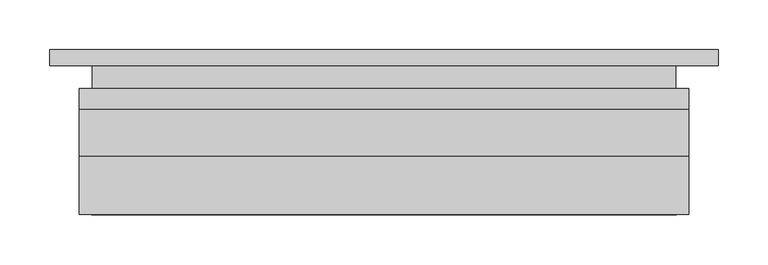
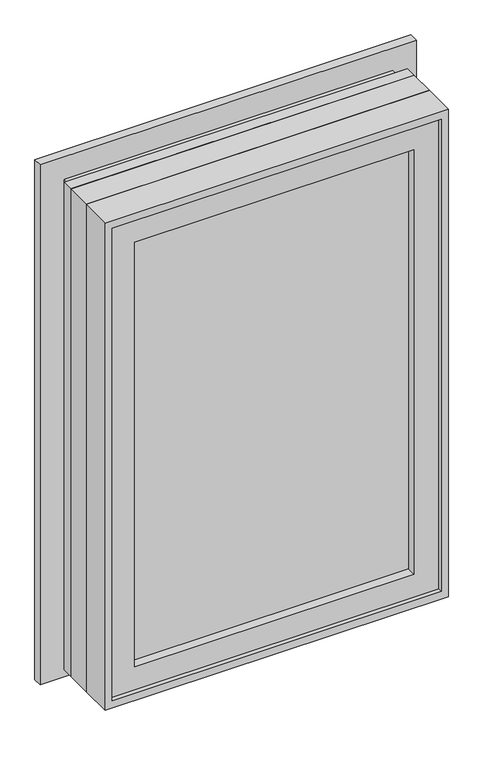
"""IFC4 building model written with IfcOpenShell, lengths in millimetres: proxy geometry, Window-Casement-Andersen-400_Series_Single : Window-Casement-Andersen-400_Series_Single."""

import ifcopenshell
import ifcopenshell.guid

model = None  # the IFC model being written
_history = None  # IfcOwnerHistory: only IFC2X3 demands one
_inside = {}  # id of a spatial element -> (the spatial element, [elements in it])
_under = {}  # id of a project, library or spatial element -> (it, [spatial elements below it])
_declared = {}  # id of a project -> (the project, [libraries it declares])
_typed = {}  # id of a type object -> (the type object, [elements of that type])
_made_of = {}  # id of a material, layer set ... -> (it, [elements and type objects made of it])


def new_model(schema):
    """Start an empty IFC model of exactly this schema.

    Asked for "IFC4X3", IfcOpenShell would pick the latest addendum, in which some entities
    have other attributes; the version numbers below select the first issue.
    IFC2X3 requires an IfcOwnerHistory on every rooted entity: one is made here for all.
    """
    global model, _history
    if schema == "IFC4X3":
        model = ifcopenshell.file(schema_version=(4, 3, 0, 0))
    else:
        model = ifcopenshell.file(schema=schema)
    _inside.clear()
    _under.clear()
    _declared.clear()
    _typed.clear()
    _made_of.clear()
    _history = None
    if model.schema == "IFC2X3":
        org = make("IfcOrganization", Name="unknown")
        user = make(
            "IfcPersonAndOrganization",
            ThePerson=make("IfcPerson", FamilyName="unknown"),
            TheOrganization=org,
        )
        app = make(
            "IfcApplication",
            ApplicationDeveloper=org,
            Version="unknown",
            ApplicationFullName="unknown",
            ApplicationIdentifier="unknown",
        )
        _history = make(
            "IfcOwnerHistory",
            OwningUser=user,
            OwningApplication=app,
            ChangeAction="ADDED",
            CreationDate=0,
        )
    return model


def make(cls, **values):
    """One entity of the class cls with the attributes given. An attribute that is None is left unset."""
    return model.create_entity(
        cls, **{name: value for name, value in values.items() if value is not None}
    )


def rooted(cls, **values):
    """An entity with a GlobalId (a new one), such as an element, a storey or a relation."""
    return make(cls, GlobalId=ifcopenshell.guid.new(), OwnerHistory=_history, **values)


def si_unit(unit_type, name, prefix=None):
    """IfcSIUnit, for example si_unit("LENGTHUNIT", "METRE", prefix="MILLI")."""
    return make("IfcSIUnit", UnitType=unit_type, Prefix=prefix, Name=name)


def assignment(units):
    """IfcUnitAssignment: the units of a project."""
    return None if units is None else make("IfcUnitAssignment", Units=units)


def point(xyz):
    """IfcCartesianPoint."""
    return None if xyz is None else make("IfcCartesianPoint", Coordinates=xyz)


def direction(xyz):
    """IfcDirection."""
    return None if xyz is None else make("IfcDirection", DirectionRatios=xyz)


def frame(location, z_axis=None, x_axis=None):
    """IfcAxis2Placement3D, a coordinate frame: its origin and axes. An axis left out is left unset."""
    return make(
        "IfcAxis2Placement3D",
        Location=point(location),
        Axis=direction(z_axis),
        RefDirection=direction(x_axis),
    )


def origin():
    """The frame at (0, 0, 0) with its axes left unset."""
    return frame((0.0, 0.0, 0.0))


def place(relative_to, where):
    """IfcLocalPlacement: puts the frame where relative to a parent placement (None: the world)."""
    return make(
        "IfcLocalPlacement", PlacementRelTo=relative_to, RelativePlacement=where
    )


def context(
    kind, dimensions, precision=None, world=None, true_north=None, identifier=None
):
    """IfcGeometricRepresentationContext, for example the 3D "Model" context."""
    return make(
        "IfcGeometricRepresentationContext",
        ContextIdentifier=identifier,
        ContextType=kind,
        CoordinateSpaceDimension=dimensions,
        Precision=precision,
        WorldCoordinateSystem=world,
        TrueNorth=true_north,
    )


def project(units=None, contexts=None):
    """IfcProject with its units and contexts."""
    return rooted(
        "IfcProject",
        Name="project",
        RepresentationContexts=contexts,
        UnitsInContext=assignment(units),
    )


def spatial(cls, under=None, at=None, **own):
    """A site, building, storey or space (cls), placed at a placement, below another one or the project."""
    s = rooted(cls, ObjectPlacement=at, **own)
    if under is not None:
        _under.setdefault(under.id(), (under, []))[1].append(s)
    return s


def polyline(points):
    """IfcPolyline through the points."""
    return make("IfcPolyline", Points=[point(p) for p in points])


def outline(outer, holes=None, kind="AREA"):
    """IfcArbitraryClosedProfileDef: a profile drawn as a closed curve; with holes, ...WithVoids."""
    if holes is None:
        return make("IfcArbitraryClosedProfileDef", ProfileType=kind, OuterCurve=outer)
    return make(
        "IfcArbitraryProfileDefWithVoids",
        ProfileType=kind,
        OuterCurve=outer,
        InnerCurves=holes,
    )


def extrude(swept, where, along, depth):
    """IfcExtrudedAreaSolid: the profile swept, set in the frame where, extruded along a direction by depth."""
    return make(
        "IfcExtrudedAreaSolid",
        SweptArea=swept,
        Position=where,
        ExtrudedDirection=direction(along),
        Depth=depth,
    )


def faces_of(points, faces, orient=None, outer=None):
    """IfcFace entities. A face is a list of loops; a loop is a list of indices into points, from 0.

    orient and outer hold one flag for each loop. By default every Orientation is true, the
    first loop of a face is its IfcFaceOuterBound and the others are IfcFaceBound.
    """
    made = []
    for i, loops in enumerate(faces):
        bounds = []
        for j, loop in enumerate(loops):
            is_outer = j == 0 if outer is None else outer[i][j]
            bounds.append(
                make(
                    "IfcFaceOuterBound" if is_outer else "IfcFaceBound",
                    Bound=make("IfcPolyLoop", Polygon=[points[k] for k in loop]),
                    Orientation=True if orient is None else orient[i][j],
                )
            )
        made.append(make("IfcFace", Bounds=bounds))
    return made


def faceted_brep(points, faces, orient=None, outer=None, voids=None):
    """IfcFacetedBrep: a solid bounded by flat faces; with voids (closed shells), ...WithVoids."""
    shared = [point(p) for p in points]
    hull = make("IfcClosedShell", CfsFaces=faces_of(shared, faces, orient, outer))
    if voids is None:
        return make("IfcFacetedBrep", Outer=hull)
    return make(
        "IfcFacetedBrepWithVoids",
        Outer=hull,
        Voids=[
            make(cls, CfsFaces=faces_of(shared, fs, o, b)) for cls, fs, o, b in voids
        ],
    )


def shape(context_of_items, identifier, shape_type, items):
    """IfcShapeRepresentation: the items that make up one representation, for example the "Body"."""
    return make(
        "IfcShapeRepresentation",
        ContextOfItems=context_of_items,
        RepresentationIdentifier=identifier,
        RepresentationType=shape_type,
        Items=items,
    )


def source(mapping_origin, context_of_items, identifier, shape_type, items):
    """IfcRepresentationMap: a shape defined once, which mapped items show again and again."""
    return make(
        "IfcRepresentationMap",
        MappingOrigin=mapping_origin,
        MappedRepresentation=shape(context_of_items, identifier, shape_type, items),
    )


def transform(
    local_origin,
    x_axis=None,
    y_axis=None,
    z_axis=None,
    scale=None,
    scale2=None,
    scale3=None,
    uniform=True,
):
    """IfcCartesianTransformationOperator3D, or its non-uniform kind. x_axis, y_axis, z_axis: its Axis1, 2, 3."""
    if uniform:
        return make(
            "IfcCartesianTransformationOperator3D",
            Axis1=direction(x_axis),
            Axis2=direction(y_axis),
            LocalOrigin=point(local_origin),
            Scale=scale,
            Axis3=direction(z_axis),
        )
    return make(
        "IfcCartesianTransformationOperator3DnonUniform",
        Axis1=direction(x_axis),
        Axis2=direction(y_axis),
        LocalOrigin=point(local_origin),
        Scale=scale,
        Axis3=direction(z_axis),
        Scale2=scale2,
        Scale3=scale3,
    )


def mapped(mapping_source, mapping_target):
    """IfcMappedItem: shows the shape of a source again, moved by a transform."""
    return make(
        "IfcMappedItem", MappingSource=mapping_source, MappingTarget=mapping_target
    )


def made_of(thing, what):
    """Note that an element or type object is made of a material, layer set ...; save() writes the relation."""
    if what is not None:
        _made_of.setdefault(what.id(), (what, []))[1].append(thing)
    return thing


def element(
    cls,
    number,
    at=None,
    inside=None,
    cuts=None,
    type_object=None,
    material=None,
    context=None,
    identifier="Body",
    shape_type=None,
    held_by="IfcProductDefinitionShape",
    body=None,
    shapes=None,
    **own,
):
    """One element of the class cls, such as IfcWall. Its Tag is "e" and its number.

    at: its placement. inside: the storey or other place that contains it. cuts: it is an
    opening in that element (IfcRelVoidsElement). A single representation is given by context,
    identifier, shape_type and body (its items); several are given by shapes. held_by: the class
    of the entity that holds the representations. save() writes the other relations.
    """
    e = rooted(cls, Tag="e%d" % number, ObjectPlacement=at, **own)
    if body is not None:
        shapes = [shape(context, identifier, shape_type, body)]
    if shapes is not None:
        e.Representation = make(held_by, Representations=shapes)
    if inside is not None:
        _inside.setdefault(inside.id(), (inside, []))[1].append(e)
    if cuts is not None:
        rooted(
            "IfcRelVoidsElement", RelatingBuildingElement=cuts, RelatedOpeningElement=e
        )
    if type_object is not None:
        _typed.setdefault(type_object.id(), (type_object, []))[1].append(e)
    return made_of(e, material)


def aggregate(whole, parts):
    """IfcRelAggregates: a whole, such as a stair, and the parts it consists of."""
    return rooted("IfcRelAggregates", RelatingObject=whole, RelatedObjects=parts)


def save(model, path):
    """Write the relations noted so far, then the file.

    IfcRelAggregates (storeys below a building ...), IfcRelContainedInSpatialStructure (elements
    in a storey), IfcRelDefinesByType, IfcRelAssociatesMaterial and IfcRelDeclares: one each for
    every whole, place, type object, material and project.
    """
    for whole, parts in _under.values():
        aggregate(whole, parts)
    for where, things in _inside.values():
        rooted(
            "IfcRelContainedInSpatialStructure",
            RelatedElements=things,
            RelatingStructure=where,
        )
    for kind, things in _typed.values():
        rooted("IfcRelDefinesByType", RelatedObjects=things, RelatingType=kind)
    for what, things in _made_of.values():
        rooted("IfcRelAssociatesMaterial", RelatedObjects=things, RelatingMaterial=what)
    for by, libraries in _declared.values():
        rooted("IfcRelDeclares", RelatingContext=by, RelatedDefinitions=libraries)
    model.write(path)


def generic_models_14e9118a(model_context):
    return source(origin(), model_context, "Body", "SolidModel", [
        extrude(outline(polyline([(-248.08815, -27.8804687), (-248.08815, -12.0054687), (248.0056, -12.0054687), (248.0056, -27.8804687), (-248.08815, -27.8804687)])), frame((0.0, 0.0, 1231.9154446), z_axis=(0.0, 0.0, 1.0), x_axis=(1.0, 0.0, 0.0)), (0.0, 0.0, 1.0), 796.925),
        extrude(outline(polyline([(2074.8779446, -292.53815), (1189.0529446, -292.53815), (1189.0529446, 292.4556), (2074.8779446, 292.4556), (2074.8779446, -292.53815)]), holes=[polyline([(2028.8404446, -248.08815), (2028.8404446, 248.0056), (1231.9154446, 248.0056), (1231.9154446, -248.08815), (2028.8404446, -248.08815)])]), frame((0.0, -44.45, 0.0), z_axis=(0.0, 1.0, 0.0), x_axis=(0.0, 0.0, 1.0)), (0.0, 0.0, 1.0), 50.8),
        faceted_brep([(-276.6314, 6.35, 2060.956), (276.6314, 6.35, 2060.956), (276.6314, 57.15, 2060.956), (-276.6314, 57.15, 2060.956), (-276.6314, 6.35, 1199.769), (-276.6314, 53.2892, 1199.769), (276.6314, 53.2892, 1199.769), (276.6314, 6.35, 1199.769), (-276.6314, 57.15, 1202.53125), (-276.6314, 53.2892, 1202.53125), (276.6314, 57.15, 1202.53125), (258.7752, 57.15, 1217.2188), (258.7752, 57.15, 2040.763), (-258.7752, 57.15, 2040.763), (-258.7752, 57.15, 1217.2188), (-258.7752, 46.175563, 1236.2942), (-258.7752, 46.175563, 1225.8587599), (-258.7752, 53.3654, 1217.2188), (-258.7752, 31.75, 2040.763), (-258.7752, 31.75, 1236.2942), (258.7752, 31.75, 2040.763), (258.7752, 31.75, 1236.2942), (254.0, 31.75, 1238.25), (254.0, 31.75, 2031.603125), (-254.0, 31.75, 2031.603125), (-254.0, 31.75, 1238.25), (-254.0, 6.35, 2031.603125), (-254.0, 6.35, 1231.138), (-254.0, 13.1318, 1238.25), (254.0, 6.35, 2031.603125), (254.0, 6.35, 1231.138), (254.0, 13.1318, 1238.25), (258.7752, 53.3654, 1217.2188), (258.7752, 46.175563, 1225.8587599), (258.7752, 46.175563, 1236.2942), (276.6314, 53.2892, 1202.53125), (-277.01875, 73.9267, 2061.36875), (277.01875, 73.9267, 2061.36875), (277.01875, 53.2892, 2061.36875), (-277.01875, 53.2892, 2061.36875), (-304.8, 53.2892, 2089.15), (304.8, 53.2892, 2089.15), (304.8, 73.9267, 2089.15), (-304.8, 73.9267, 2089.15), (277.01875, 73.9267, 1202.53125), (277.01875, 53.2892, 1202.53125), (304.8, 53.2892, 1174.75), (304.8, 73.9267, 1174.75), (-277.01875, 73.9267, 1202.53125), (-277.01875, 53.2892, 1202.53125), (-304.8, 53.2892, 1174.75), (-304.8, 73.9267, 1174.75)], [[[0, 1, 2, 3]], [[4, 5, 6, 7]], [[3, 8, 9, 5, 4, 0]], [[2, 10, 8, 3], [11, 12, 13, 14]], [[15, 16, 17, 14, 13, 18, 19]], [[19, 18, 20, 21], [22, 23, 24, 25]], [[25, 24, 26, 27, 28]], [[7, 1, 0, 4], [27, 26, 29, 30]], [[31, 30, 29, 23, 22]], [[21, 20, 12, 11, 32, 33, 34]], [[1, 7, 6, 35, 10, 2]], [[25, 28, 31, 22]], [[30, 31, 28, 27]], [[15, 19, 21, 34]], [[34, 33, 16, 15]], [[33, 32, 17, 16]], [[14, 17, 32, 11]], [[12, 20, 18, 13]], [[23, 29, 26, 24]], [[36, 37, 38, 39]], [[40, 41, 42, 43]], [[37, 44, 45, 38]], [[41, 46, 47, 42]], [[44, 48, 49, 9, 8, 10, 35, 45]], [[46, 50, 51, 47]], [[39, 49, 48, 36]], [[42, 47, 51, 43], [36, 48, 44, 37]], [[43, 51, 50, 40]], [[40, 50, 46, 41], [38, 45, 35, 6, 5, 9, 49, 39]]]),
        extrude(outline(polyline([(2089.15, -304.8), (1174.75, -304.8), (1174.75, 304.8), (2089.15, 304.8), (2089.15, -304.8)]), holes=[polyline([(2060.956, -276.6314), (2060.956, 276.6314), (1199.769, 276.6314), (1199.769, -276.6314), (2060.956, -276.6314)])]), frame((0.0, 6.35, 0.0), z_axis=(0.0, 1.0, 0.0), x_axis=(0.0, 0.0, 1.0)), (0.0, 0.0, 1.0), 46.9392),
        extrude(outline(polyline([(2089.15, -304.8), (1174.75, -304.8), (1174.75, 304.8), (2089.15, 304.8), (2089.15, -304.8)]), holes=[polyline([(2074.8470554, -292.4556), (2074.8470554, 292.4556), (1189.0529446, 292.4556), (1189.0529446, -292.4556), (2074.8470554, -292.4556)])]), frame((0.0, -52.3748, 0.0), z_axis=(0.0, 1.0, 0.0), x_axis=(0.0, 0.0, 1.0)), (0.0, 0.0, 1.0), 58.7248),
        extrude(outline(polyline([(2118.51875, 334.16875), (2118.51875, -334.16875), (1142.619, -334.16875), (1142.619, 334.16875), (2118.51875, 334.16875)]), holes=[polyline([(2061.36875, 277.01875), (1199.769, 277.01875), (1199.769, -277.01875), (2061.36875, -277.01875), (2061.36875, 277.01875)])]), frame((0.0, 96.8375, 0.0), z_axis=(0.0, 1.0, 0.0), x_axis=(0.0, 0.0, 1.0)), (0.0, 0.0, 1.0), 15.875),
        extrude(outline(polyline([(2076.45, 292.1), (2076.45, -292.1), (1187.45, -292.1), (1187.45, 292.1), (2076.45, 292.1)]), holes=[polyline([(2061.36875, 277.01875), (1199.769, 277.01875), (1199.769, -277.01875), (2061.36875, -277.01875), (2061.36875, 277.01875)])]), frame((0.0, 53.18125, 0.0), z_axis=(0.0, 1.0, 0.0), x_axis=(0.0, 0.0, 1.0)), (0.0, 0.0, 1.0), 43.65625),
    ])


if __name__ == "__main__":
    model = new_model("IFC4")
    model_context = context("Model", 3, world=origin())
    ifc_project = project(units=[si_unit("LENGTHUNIT", "METRE", prefix="MILLI")], contexts=[model_context])
    site = spatial("IfcSite", under=ifc_project)
    building = spatial("IfcBuilding", under=site)
    placement = place(None, origin())
    generic_models_shape = generic_models_14e9118a(model_context)
    element("IfcBuildingElementProxy", 1, Name="Window-Casement-Andersen-400_Series_Single : Window-Casement-Andersen-400_Series_Single", ObjectType="Window-Casement-Andersen-400_Series_Single : Window-Casement-Andersen-400_Series_Single", at=placement, inside=building, context=model_context, shape_type="MappedRepresentation", body=[
        mapped(generic_models_shape, transform((0.0, 0.0, 0.0), x_axis=(1.0, 0.0, 0.0), y_axis=(0.0, 1.0, 0.0), z_axis=(0.0, 0.0, 1.0))),
    ])
    save(model, "model.ifc")

# Revit data of these elements
# Type "Window-Casement-Andersen-400_Series_Single : Window-Casement-Andersen-400_Series_Single"
#   Type Mark = "2"
#   Learn About These Parameters = "http://www.andersenwindows.com/for-professionals/cad-symbols-bim-support-window-doors/bim-support"
#   ..Jamb Condition Number 1 = "Extension Jamb Only"
#   ..Jamb Condition Number 2 = "Narrow Drywall Return"
#   ..Jamb Condition Number 3 = "Wide Drywall Return"
#   Available Grille Bar Sizes = "3/4'', 7/8'', 1 1/8'', 2 1/4''"
#   Between Glass Grille Bar Sizes = "3/4'', 1''"
#   ..Pattern Number 1 = "Colonial"
#   ..Pattern Number 2 = "Modified Colonial"
#   ..Pattern Number 3 = "Prairie"
#   ..Pattern Number 4 = "Short Fractional"
#   ..Pattern Number 5 = "Tall Fractional"
#   ..Exterior Trim Number 0 = "No Exterior Trim"
#   ..Exterior Trim Number 1 = "Brick Mould"
#   ..Exterior Trim Number 2 = "3 1/2'' Flat Casing"
#   ..Exterior Trim Number 3 = "4 1/2'' Flat Casing"
#   URL = "www.andersenwindows.com"
#   Type Comments = "Vinyl-clad wood casement window"
#   Product Documentation Link = "https://www.andersenwindows.com/windows-and-doors/windows/casement-windows/400-series-casement-window/"
#   Model = "400-Series Casement"
#   Manufacturer = "Andersen Corporation"
#   Family Version = "01.01.19"
#   Designation = "CMT"
#   Description = "Vinyl-clad wood casement window"
#   Assembly Code = "B2020100"
#   XPanelWidth = 1' - 11 1/32"
#   XPanelHeight = 2' - 10 7/8"
#   Width = 2' - 0"
#   Visual Light Transmittance = 0.48
#   Thermal Resistance (R) = 0.628713 (stored number, unit not read)
#   Solar Heat Gain Coefficient = 0.21
#   Rough Width = 2' - 0 1/2"
#   Rough Height = 3' - 0 1/2"
#   Height = 3' - 0"
#   Heat Transfer Coefficient (U) = 1.58991 (stored number, unit not read)
#   Grille Bar Size = 0' - 0 7/8"
#   xjamb S1 [instance default] = 0' - 1 23/32"
#   sill nose1 = 0' - 1 13/16"
#   sill nose 2 = 0' - 1 15/16"
#   casingS2 = 0' - 0 3/16"
#   casingS1 = 0' - 0 3/16"
#   casing4 = 0' - 4 1/4"
#   casing3 = 0' - 0 1/2"
#   casing2 = 0' - 0 7/8"
#   casing1 = 0' - 0 1/4"
#   Xjamb 2 = 0' - 0 1/2"
#   Xjamb 1 = 0' - 1 3/32"
#   Wall Thickness [instance default] = 0' - 6"
#   Wall Depth [instance default] = 0' - 4 9/16"
#   Void Offset 2 = 0' - 0"
#   Void Offset 1 = 0' - 0"
#   Void Depth [instance default] = 0' - 2 7/16"
#   VGB DLO = 0' - 5.91667"
#   TS V DLO = 2' - 7 3/8"
#   TS V Bar Length = 2' - 7 3/8"
#   TS SH DLO = 1' - 6 1/16"
#   TS HGB DLO = 0' - 9 7/8"
#   Step Jamb2 = 0' - 0 13/16"
#   Step Jamb1 = 0' - 1 1/8"
#   Sill Stop Dim [instance default] = 0' - 2 1/2"
#   SGO = 0' - 2 1/4"
#   Rough Opening Offset = 0' - 0 1/4"
#   Plan Exterior Mask 2 [instance default] = 0' - 1 3/8"
#   Plan Exterior Mask [instance default] = 0' - 1 1/16"
#   Masonry Width = 2' - 0 1/2"
#   Masonry Opening Offset = 0' - 0 1/4"
#   Masonry Height = 3' - 0 1/2"
#   JGO = 0' - 2 1/4"
#   Interior Casing Size = 0' - 2 1/4"
#   Horizontal Craftsman Bar Size = 0' - 0 7/8"
#   Head Stop Dim [instance default] = 0' - 2 17/64"
#   HGO = 0' - 2 3/8"
#   H DLO = 1' - 7 1/2"
#   Default Sill Height = 3' - 10"
#   Coarse Plan [instance default] = 0' - 4 9/16"
#   TFL = 2
#   TFB = 1
#   LWide = 3
#   Fractional Lights Wide = 3
#   Fractional Lights High = 5
#   Enter Jamb Condition = 1
#   Interior Casing = yes
#   Enter Pattern Number = 1
#   . . Lights Wide = 3
#   . . Lights High = 3
#   Extension Jamb = yes
#   Enter Exterior Trim Number = 0
#   Interior Grille Bar = yes
#   Exterior Grille Bar = yes
#   Between Glass Grille Bar = yes
#   xjamb Visibility [instance default] = yes
#   VeriLock Sensor [instance default] = no
#   V Bars = 2
#   TS S V = no
#   TS S H Craftsman = no
#   TS S H = no
#   TS M V = yes
#   TS M H = yes
#   TS H Bars = 2
#   Step Visibility = no
#   Push Out Stop Visibility [instance default] = no
#   Plan Exterior Mask Visibility [instance default] = yes
#   Nail Fin Visibility = yes
#   Interior Trim Visibility = yes
#   Crank Out Stop Visibility [instance default] = yes
#   Casing Visibility = no
#   Bar Center Line = 2
#   Glazing Material = DOUBLE HUNG WINDOWS
#   Exterior Unit Finish = Vinyl - Andersen - White
#   Interior Material = Wood - Andersen - Pine
#   Exterior Trim Finish = Fibrex Composite - Andersen - White
#   Between Glass Grille Bar Finish = Stainless Steel - Andersen - Standard
#   Wall Closure = (empty or 0)
# Element 1 (IfcBuildingElementProxy, "Window-Casement-Andersen-400_Series_Single : Window-Casement-Andersen-400_Series_Single")
#   Wall Thickness = 0' - 7 5/8"
#   Void Depth = 0' - 4 1/16"
#   Plan Exterior Mask 2 = 0' - 3"
#   Materials on its faces: "Wood - Andersen - Pine", "Vinyl - Andersen - White", "DOUBLE HUNG WINDOWS"
# Materials
#   "DOUBLE HUNG WINDOWS": class "Glass", colour RGB 236 240 239, transparency 0.85, Cost = 0
#   "Vinyl - Andersen - White": class "Plastic", colour RGB 241 238 228, transparency 0, Description = "White vinyl finish", Cost = 0
#   "Wood - Andersen - Pine": class "Wood", colour RGB 235 199 148, transparency 0, Description = "Pinus Echinata", Cost = 0
#   "Fibrex Composite - Andersen - White": class "Plastic", colour RGB 241 238 228, transparency 0, Manufacturer = "Andersen", Description = "Wood fiber and thermoplastic polymer composite material", Cost = 0
#   "Stainless Steel - Andersen - Standard": class "Metal", colour RGB 149 149 150, transparency 0, Cost = 0
